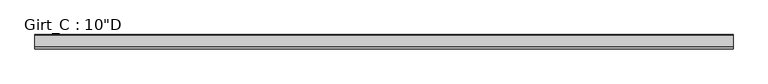
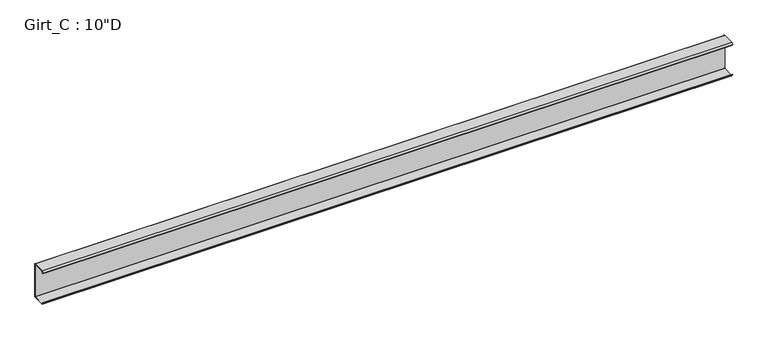
"""IFC4 building model written with IfcOpenShell, lengths in millimetres: beam geometry."""

from ifc_helpers import new_model, si_unit, point, frame, frame_2d, origin, place, context, project, spatial, polyline, circle_curve, trimmed, segment, composite_curve, outline, extrude, source, transform, mapped, element, save


def beam_7096158d(model_context):
    return source(origin(), model_context, "Body", "SweptSolid", [
        extrude(outline(composite_curve([segment(polyline([(-87.5109375, 127.0), (-3.3734375, 127.0)]), True, "CONTINUOUS"), segment(trimmed(circle_curve(frame_2d((-3.3734375, 122.2375)), 4.7625), [point((-3.3734375, 127.0))], [point((1.3890625, 122.2375))], False, "CARTESIAN"), True, "CONTINUOUS"), segment(polyline([(1.3890625, 122.2375), (1.3890625, -122.2375)]), True, "CONTINUOUS"), segment(trimmed(circle_curve(frame_2d((-3.3734375, -122.2375)), 4.7625), [point((1.3890625, -122.2375))], [point((-3.3734375, -127.0))], False, "CARTESIAN"), True, "CONTINUOUS"), segment(polyline([(-3.3734375, -127.0), (-87.5109375, -127.0), (-99.7792647, -112.379177), (-97.6510975, -110.5934327), (-86.2154765, -124.221875), (-3.2694106, -124.221875)]), True, "CONTINUOUS"), segment(trimmed(circle_curve(frame_2d((-3.3748024, -122.2389339)), 1.9857399), [point((-3.2694106, -124.221875))], [point((-1.3890625, -122.2389339))], True, "CARTESIAN"), True, "CONTINUOUS"), segment(polyline([(-1.3890625, -122.2389339), (-1.3890625, 122.2381931)]), True, "CONTINUOUS"), segment(trimmed(circle_curve(frame_2d((-3.3741066, 122.2381931)), 1.9850441), [point((-1.3890625, 122.2381931))], [point((-3.3005807, 124.221875))], True, "CARTESIAN"), True, "CONTINUOUS"), segment(polyline([(-3.3005807, 124.221875), (-86.2154765, 124.221875), (-97.6278742, 110.621109), (-99.7560415, 112.4068534), (-87.5109375, 127.0)]), True, "CONTINUOUS")], self_intersect=False)), frame((-2501.6206, 0.0, 0.0), z_axis=(1.0, 0.0, 0.0), x_axis=(0.0, 1.0, 0.0)), (0.0, 0.0, 1.0), 4939.538),
    ])


if __name__ == "__main__":
    model = new_model("IFC4")
    model_context = context("Model", 3, world=origin())
    ifc_project = project(units=[si_unit("LENGTHUNIT", "METRE", prefix="MILLI")], contexts=[model_context])
    site = spatial("IfcSite", under=ifc_project)
    building = spatial("IfcBuilding", under=site)
    placement = place(None, origin())
    beam_shape = beam_7096158d(model_context)
    element("IfcBeam", 1, ObjectType="Girt_C : 10\"D", at=placement, inside=building, context=model_context, shape_type="MappedRepresentation", body=[
        mapped(beam_shape, transform((0.0, 0.0, 0.0), x_axis=(1.0, 0.0, 0.0), y_axis=(0.0, 1.0, 0.0), z_axis=(0.0, 0.0, 1.0))),
    ])
    save(model, "model.ifc")

# Revit data of these elements
# Type "Girt_C : 10\"D"
#   half leg = 0' - 1 3/4"
#   Web_Thickness = 0' - 0 7/64"
#   Length [instance default] = 10' - 0"
#   Leg_1 = 0' - 3 1/2"
#   Height = 0' - 10"
#   Structural Material [instance default] = none
# Element 1 (IfcBeam, "Girt_C : 10\"D")
#   Structural Material = STRUCTURAL STEEL - SEE STRUCT. DWGS
#   Materials on its faces: "STRUCTURAL STEEL - SEE STRUCT. DWGS"
# Materials
#   "STRUCTURAL STEEL - SEE STRUCT. DWGS": class "Metal", colour RGB 137 146 153, transparency 0, Description = "Steel, mill finish", Cost = 0
